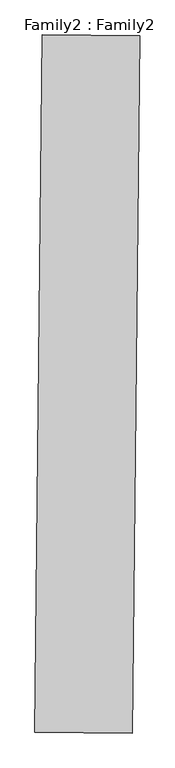
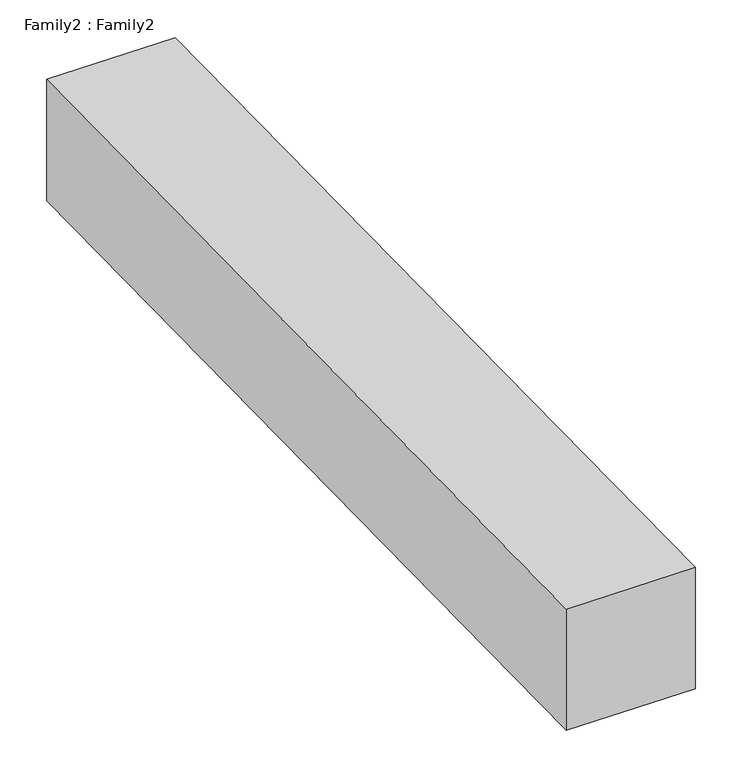
"""IFC4 building model written with IfcOpenShell, lengths in millimetres: proxy geometry, Family2 : Family2."""

from ifc_helpers import new_model, si_unit, origin, place, context, project, spatial, faceted_brep, source, transform, mapped, element, save


def family2_family2_d2316618(model_context):
    return source(origin(), model_context, "Body", "Brep", [
        faceted_brep([(-3950.9511552, -6789.210751, 1.0945136), (-3950.9511552, -6789.210751, 201.0945136), (-3935.8916393, -5358.3893716, 202.060409), (-3935.8916393, -5358.3893716, 2.060409), (-3750.9599652, -6791.0879636, 201.0945136), (-3735.9004493, -5360.2665843, 202.060409), (-3750.9599652, -6791.0879636, 1.0945136), (-3735.9004493, -5360.2665843, 2.060409)], [[[0, 1, 2, 3]], [[1, 4, 5, 2]], [[4, 6, 7, 5]], [[6, 0, 3, 7]], [[3, 2, 5, 7]], [[0, 6, 4, 1]]]),
    ])


if __name__ == "__main__":
    model = new_model("IFC4")
    model_context = context("Model", 3, world=origin())
    ifc_project = project(units=[si_unit("LENGTHUNIT", "METRE", prefix="MILLI")], contexts=[model_context])
    site = spatial("IfcSite", under=ifc_project)
    building = spatial("IfcBuilding", under=site)
    placement = place(None, origin())
    family2_family2_shape = family2_family2_d2316618(model_context)
    element("IfcBuildingElementProxy", 1, Name="Family2 : Family2", ObjectType="Family2 : Family2", at=placement, inside=building, context=model_context, shape_type="MappedRepresentation", body=[
        mapped(family2_family2_shape, transform((0.0, 0.0, 0.0), x_axis=(1.0, 0.0, 0.0), y_axis=(0.0, 1.0, 0.0), z_axis=(0.0, 0.0, 1.0))),
    ])
    save(model, "model.ifc")

# Revit data of these elements
# Type "Family2 : Family2"
#   Default Elevation = 0
